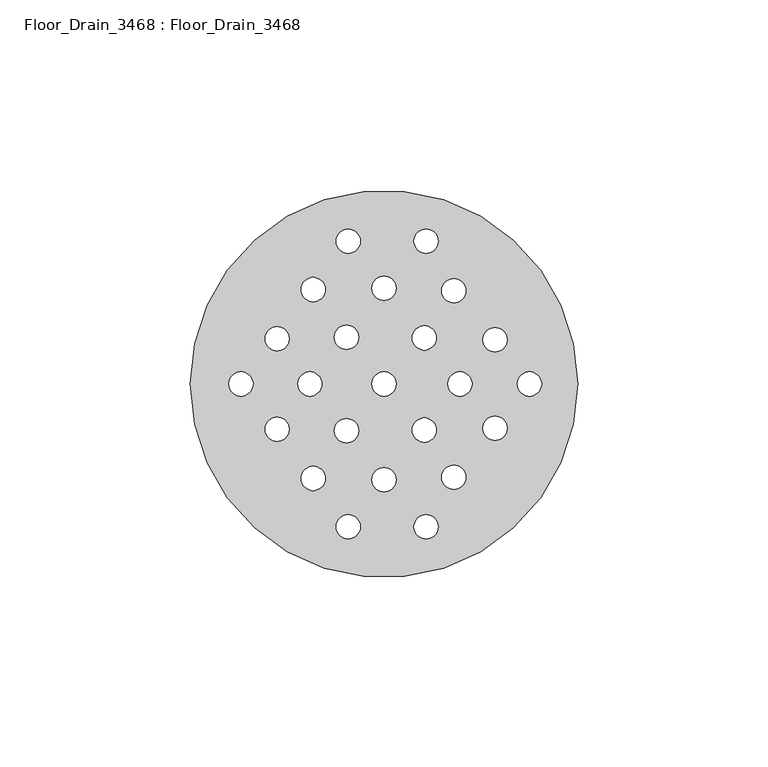
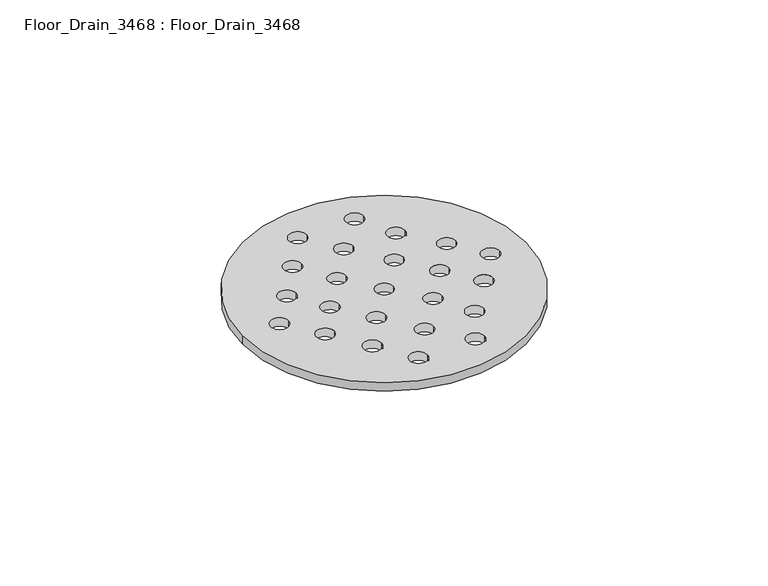
"""IFC4 building model written with IfcOpenShell, lengths in millimetres: flow terminal geometry, Floor_Drain_3468 : Floor_Drain_3468."""

from ifc_helpers import new_model, si_unit, point, frame_2d, origin, origin_with_axes, origin_2d, place, context, project, spatial, circle_curve, trimmed, segment, composite_curve, outline, extrude, source, transform, mapped, element, save


def floor_drain_3468_floor_drain_3468_976f3ea6(model_context):
    return source(origin(), model_context, "Body", "SweptSolid", [
        extrude(outline(composite_curve([segment(trimmed(circle_curve(origin_2d(), 50.8), [point((-50.8, 0.0))], [point((50.8, 0.0))], False, "CARTESIAN"), True, "CONTINUOUS"), segment(trimmed(circle_curve(origin_2d(), 50.8), [point((50.8, 0.0))], [point((-50.8, 0.0))], False, "CARTESIAN"), True, "CONTINUOUS")], self_intersect=False), holes=[composite_curve([segment(trimmed(circle_curve(frame_2d((-37.5575401, 0.0)), 3.175), [point((-40.7325401, 0.0))], [point((-34.3825401, 0.0))], True, "CARTESIAN"), True, "CONTINUOUS"), segment(trimmed(circle_curve(frame_2d((-37.5575401, 0.0)), 3.175), [point((-34.3825401, 0.0))], [point((-40.7325401, 0.0))], True, "CARTESIAN"), True, "CONTINUOUS")], self_intersect=False), composite_curve([segment(trimmed(circle_curve(origin_2d(), 3.175), [point((-3.175, 0.0))], [point((3.175, 0.0))], True, "CARTESIAN"), True, "CONTINUOUS"), segment(trimmed(circle_curve(origin_2d(), 3.175), [point((3.175, 0.0))], [point((-3.175, 0.0))], True, "CARTESIAN"), True, "CONTINUOUS")], self_intersect=False), composite_curve([segment(trimmed(circle_curve(frame_2d((38.1724441, 0.0)), 3.175), [point((34.9974441, 0.0))], [point((41.3474441, 0.0))], True, "CARTESIAN"), True, "CONTINUOUS"), segment(trimmed(circle_curve(frame_2d((38.1724441, 0.0)), 3.175), [point((41.3474441, 0.0))], [point((34.9974441, 0.0))], True, "CARTESIAN"), True, "CONTINUOUS")], self_intersect=False), composite_curve([segment(trimmed(circle_curve(frame_2d((19.9297961, 0.0)), 3.175), [point((16.7547961, 0.0))], [point((23.1047961, 0.0))], True, "CARTESIAN"), True, "CONTINUOUS"), segment(trimmed(circle_curve(frame_2d((19.9297961, 0.0)), 3.175), [point((23.1047961, 0.0))], [point((16.7547961, 0.0))], True, "CARTESIAN"), True, "CONTINUOUS")], self_intersect=False), composite_curve([segment(trimmed(circle_curve(frame_2d((-19.4681917, 0.0)), 3.175), [point((-22.6431917, 0.0))], [point((-16.2931917, 0.0))], True, "CARTESIAN"), True, "CONTINUOUS"), segment(trimmed(circle_curve(frame_2d((-19.4681917, 0.0)), 3.175), [point((-16.2931917, 0.0))], [point((-22.6431917, 0.0))], True, "CARTESIAN"), True, "CONTINUOUS")], self_intersect=False), composite_curve([segment(trimmed(circle_curve(frame_2d((-28.0529672, -11.8979532)), 3.175), [point((-31.2279672, -11.8979532))], [point((-24.8779672, -11.8979532))], True, "CARTESIAN"), True, "CONTINUOUS"), segment(trimmed(circle_curve(frame_2d((-28.0529672, -11.8979532)), 3.175), [point((-24.8779672, -11.8979532))], [point((-31.2279672, -11.8979532))], True, "CARTESIAN"), True, "CONTINUOUS")], self_intersect=False), composite_curve([segment(trimmed(circle_curve(frame_2d((-9.8375714, -12.2318045)), 3.175), [point((-13.0125714, -12.2318045))], [point((-6.6625714, -12.2318045))], True, "CARTESIAN"), True, "CONTINUOUS"), segment(trimmed(circle_curve(frame_2d((-9.8375714, -12.2318045)), 3.175), [point((-6.6625714, -12.2318045))], [point((-13.0125714, -12.2318045))], True, "CARTESIAN"), True, "CONTINUOUS")], self_intersect=False), composite_curve([segment(trimmed(circle_curve(frame_2d((10.5785227, -12.078505)), 3.175), [point((7.4035227, -12.078505))], [point((13.7535227, -12.078505))], True, "CARTESIAN"), True, "CONTINUOUS"), segment(trimmed(circle_curve(frame_2d((10.5785227, -12.078505)), 3.175), [point((13.7535227, -12.078505))], [point((7.4035227, -12.078505))], True, "CARTESIAN"), True, "CONTINUOUS")], self_intersect=False), composite_curve([segment(trimmed(circle_curve(frame_2d((29.1277698, -11.6186063)), 3.175), [point((25.9527698, -11.6186063))], [point((32.3027698, -11.6186063))], True, "CARTESIAN"), True, "CONTINUOUS"), segment(trimmed(circle_curve(frame_2d((29.1277698, -11.6186063)), 3.175), [point((32.3027698, -11.6186063))], [point((25.9527698, -11.6186063))], True, "CARTESIAN"), True, "CONTINUOUS")], self_intersect=False), composite_curve([segment(trimmed(circle_curve(frame_2d((-18.5756465, -24.8023687)), 3.175), [point((-21.7506465, -24.8023687))], [point((-15.4006465, -24.8023687))], True, "CARTESIAN"), True, "CONTINUOUS"), segment(trimmed(circle_curve(frame_2d((-18.5756465, -24.8023687)), 3.175), [point((-15.4006465, -24.8023687))], [point((-21.7506465, -24.8023687))], True, "CARTESIAN"), True, "CONTINUOUS")], self_intersect=False), composite_curve([segment(trimmed(circle_curve(frame_2d((0.0, -25.1089678)), 3.175), [point((-3.175, -25.1089678))], [point((3.175, -25.1089678))], True, "CARTESIAN"), True, "CONTINUOUS"), segment(trimmed(circle_curve(frame_2d((0.0, -25.1089678)), 3.175), [point((3.175, -25.1089678))], [point((-3.175, -25.1089678))], True, "CARTESIAN"), True, "CONTINUOUS")], self_intersect=False), composite_curve([segment(trimmed(circle_curve(frame_2d((18.3150439, -24.4957696)), 3.175), [point((15.1400439, -24.4957696))], [point((21.4900439, -24.4957696))], True, "CARTESIAN"), True, "CONTINUOUS"), segment(trimmed(circle_curve(frame_2d((18.3150439, -24.4957696)), 3.175), [point((21.4900439, -24.4957696))], [point((15.1400439, -24.4957696))], True, "CARTESIAN"), True, "CONTINUOUS")], self_intersect=False), composite_curve([segment(trimmed(circle_curve(frame_2d((-9.4049249, -37.4989803)), 3.175), [point((-12.5799249, -37.4989803))], [point((-6.2299249, -37.4989803))], True, "CARTESIAN"), True, "CONTINUOUS"), segment(trimmed(circle_curve(frame_2d((-9.4049249, -37.4989803)), 3.175), [point((-6.2299249, -37.4989803))], [point((-12.5799249, -37.4989803))], True, "CARTESIAN"), True, "CONTINUOUS")], self_intersect=False), composite_curve([segment(trimmed(circle_curve(frame_2d((11.0384214, -37.5262324)), 3.175), [point((7.8634214, -37.5262324))], [point((14.2134214, -37.5262324))], True, "CARTESIAN"), True, "CONTINUOUS"), segment(trimmed(circle_curve(frame_2d((11.0384214, -37.5262324)), 3.175), [point((14.2134214, -37.5262324))], [point((7.8634214, -37.5262324))], True, "CARTESIAN"), True, "CONTINUOUS")], self_intersect=False), composite_curve([segment(trimmed(circle_curve(frame_2d((-28.0529672, 11.8979532)), 3.175), [point((-31.2279672, 11.8979532))], [point((-24.8779672, 11.8979532))], True, "CARTESIAN"), True, "CONTINUOUS"), segment(trimmed(circle_curve(frame_2d((-28.0529672, 11.8979532)), 3.175), [point((-24.8779672, 11.8979532))], [point((-31.2279672, 11.8979532))], True, "CARTESIAN"), True, "CONTINUOUS")], self_intersect=False), composite_curve([segment(trimmed(circle_curve(frame_2d((-9.8375714, 12.2318045)), 3.175), [point((-13.0125714, 12.2318045))], [point((-6.6625714, 12.2318045))], True, "CARTESIAN"), True, "CONTINUOUS"), segment(trimmed(circle_curve(frame_2d((-9.8375714, 12.2318045)), 3.175), [point((-6.6625714, 12.2318045))], [point((-13.0125714, 12.2318045))], True, "CARTESIAN"), True, "CONTINUOUS")], self_intersect=False), composite_curve([segment(trimmed(circle_curve(frame_2d((10.5785227, 12.078505)), 3.175), [point((7.4035227, 12.078505))], [point((13.7535227, 12.078505))], True, "CARTESIAN"), True, "CONTINUOUS"), segment(trimmed(circle_curve(frame_2d((10.5785227, 12.078505)), 3.175), [point((13.7535227, 12.078505))], [point((7.4035227, 12.078505))], True, "CARTESIAN"), True, "CONTINUOUS")], self_intersect=False), composite_curve([segment(trimmed(circle_curve(frame_2d((29.1277698, 11.6186063)), 3.175), [point((25.9527698, 11.6186063))], [point((32.3027698, 11.6186063))], True, "CARTESIAN"), True, "CONTINUOUS"), segment(trimmed(circle_curve(frame_2d((29.1277698, 11.6186063)), 3.175), [point((32.3027698, 11.6186063))], [point((25.9527698, 11.6186063))], True, "CARTESIAN"), True, "CONTINUOUS")], self_intersect=False), composite_curve([segment(trimmed(circle_curve(frame_2d((-18.5756465, 24.8023687)), 3.175), [point((-21.7506465, 24.8023687))], [point((-15.4006465, 24.8023687))], True, "CARTESIAN"), True, "CONTINUOUS"), segment(trimmed(circle_curve(frame_2d((-18.5756465, 24.8023687)), 3.175), [point((-15.4006465, 24.8023687))], [point((-21.7506465, 24.8023687))], True, "CARTESIAN"), True, "CONTINUOUS")], self_intersect=False), composite_curve([segment(trimmed(circle_curve(frame_2d((0.0, 25.1089678)), 3.175), [point((-3.175, 25.1089678))], [point((3.175, 25.1089678))], True, "CARTESIAN"), True, "CONTINUOUS"), segment(trimmed(circle_curve(frame_2d((0.0, 25.1089678)), 3.175), [point((3.175, 25.1089678))], [point((-3.175, 25.1089678))], True, "CARTESIAN"), True, "CONTINUOUS")], self_intersect=False), composite_curve([segment(trimmed(circle_curve(frame_2d((18.3150439, 24.4957696)), 3.175), [point((15.1400439, 24.4957696))], [point((21.4900439, 24.4957696))], True, "CARTESIAN"), True, "CONTINUOUS"), segment(trimmed(circle_curve(frame_2d((18.3150439, 24.4957696)), 3.175), [point((21.4900439, 24.4957696))], [point((15.1400439, 24.4957696))], True, "CARTESIAN"), True, "CONTINUOUS")], self_intersect=False), composite_curve([segment(trimmed(circle_curve(frame_2d((-9.4049249, 37.4989803)), 3.175), [point((-12.5799249, 37.4989803))], [point((-6.2299249, 37.4989803))], True, "CARTESIAN"), True, "CONTINUOUS"), segment(trimmed(circle_curve(frame_2d((-9.4049249, 37.4989803)), 3.175), [point((-6.2299249, 37.4989803))], [point((-12.5799249, 37.4989803))], True, "CARTESIAN"), True, "CONTINUOUS")], self_intersect=False), composite_curve([segment(trimmed(circle_curve(frame_2d((11.0384214, 37.5262324)), 3.175), [point((7.8634214, 37.5262324))], [point((14.2134214, 37.5262324))], True, "CARTESIAN"), True, "CONTINUOUS"), segment(trimmed(circle_curve(frame_2d((11.0384214, 37.5262324)), 3.175), [point((14.2134214, 37.5262324))], [point((7.8634214, 37.5262324))], True, "CARTESIAN"), True, "CONTINUOUS")], self_intersect=False)]), origin_with_axes(), (0.0, 0.0, 1.0), 3.175),
    ])


if __name__ == "__main__":
    model = new_model("IFC4")
    model_context = context("Model", 3, world=origin())
    ifc_project = project(units=[si_unit("LENGTHUNIT", "METRE", prefix="MILLI")], contexts=[model_context])
    site = spatial("IfcSite", under=ifc_project)
    building = spatial("IfcBuilding", under=site)
    placement = place(None, origin())
    floor_drain_3468_floor_drain_3468_shape = floor_drain_3468_floor_drain_3468_976f3ea6(model_context)
    element("IfcFlowTerminal", 1, ObjectType="Floor_Drain_3468 : Floor_Drain_3468", at=placement, inside=building, context=model_context, shape_type="MappedRepresentation", body=[
        mapped(floor_drain_3468_floor_drain_3468_shape, transform((0.0, 0.0, 0.0), x_axis=(1.0, 0.0, 0.0), y_axis=(0.0, 1.0, 0.0), z_axis=(0.0, 0.0, 1.0))),
    ])
    save(model, "model.ifc")

# Revit data of these elements
# Type "Floor_Drain_3468 : Floor_Drain_3468"
#   Drain Material [instance default] = Default
# Element 1 (IfcFlowTerminal, "Floor_Drain_3468 : Floor_Drain_3468")
#   Materials on its faces: "Default"
# Materials
#   "Default": class "Miscellaneous", colour RGB 127 127 127, transparency 0, Cost = 0
